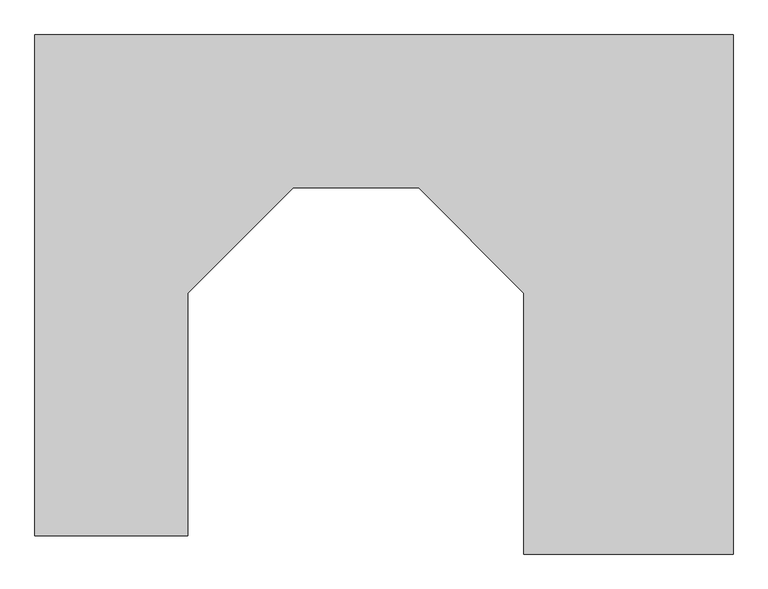
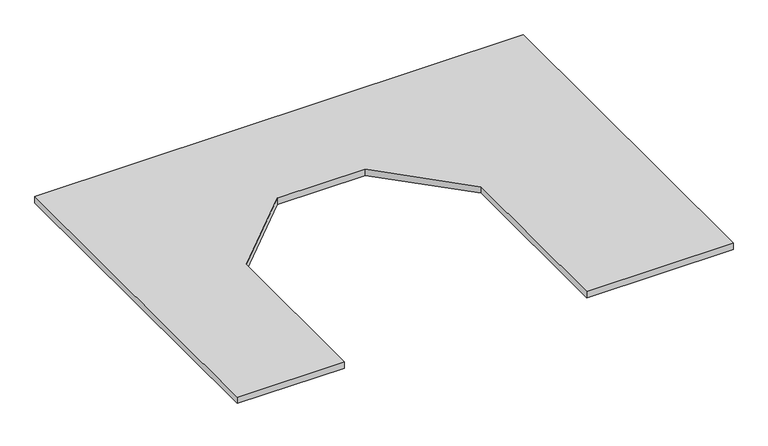
"""IFC4 building model written with IfcOpenShell, lengths in millimetres: furniture geometry, Office penisula : Office penisula."""

from ifc_helpers import new_model, si_unit, frame, origin, place, context, project, spatial, polyline, outline, extrude, source, transform, mapped, element, save


def furniture_9177ae0c(model_context):
    return source(origin(), model_context, "Body", "SweptSolid", [
        extrude(outline(polyline([(-5456.2375, 16527.4625), (-5456.2375, 15560.675), (-6065.8375, 15560.675), (-6065.8375, 17556.1625), (-3283.6387882, 17556.1625), (-3283.6387882, 15487.4834432), (-4118.0047569, 15487.4834432), (-4118.0047569, 16527.4625), (-4537.1047569, 16946.5625), (-5037.1375, 16946.5625), (-5456.2375, 16527.4625)])), frame((0.0, 0.0, 647.7), z_axis=(0.0, 0.0, 1.0), x_axis=(1.0, 0.0, 0.0)), (0.0, 0.0, 1.0), 38.1),
    ])


if __name__ == "__main__":
    model = new_model("IFC4")
    model_context = context("Model", 3, world=origin())
    ifc_project = project(units=[si_unit("LENGTHUNIT", "METRE", prefix="MILLI")], contexts=[model_context])
    site = spatial("IfcSite", under=ifc_project)
    building = spatial("IfcBuilding", under=site)
    placement = place(None, origin())
    furniture_shape = furniture_9177ae0c(model_context)
    element("IfcFurniture", 1, ObjectType="Office penisula : Office penisula", at=placement, inside=building, context=model_context, shape_type="MappedRepresentation", body=[
        mapped(furniture_shape, transform((0.0, 0.0, 0.0), x_axis=(1.0, 0.0, 0.0), y_axis=(0.0, 1.0, 0.0), z_axis=(0.0, 0.0, 1.0))),
    ])
    save(model, "model.ifc")

# Revit data of these elements
# Type "Office penisula : Office penisula"
#   COBie.Type = no
# Element 1 (IfcFurniture, "Office penisula : Office penisula")
#   Materials on its faces: "Green Laminate"
# Materials
#   "Green Laminate": class "Generic", colour RGB 57 96 54, transparency 0, Cost = 0
